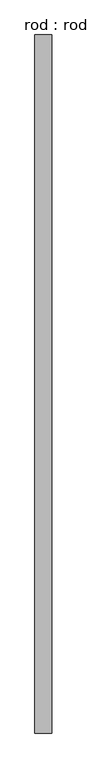
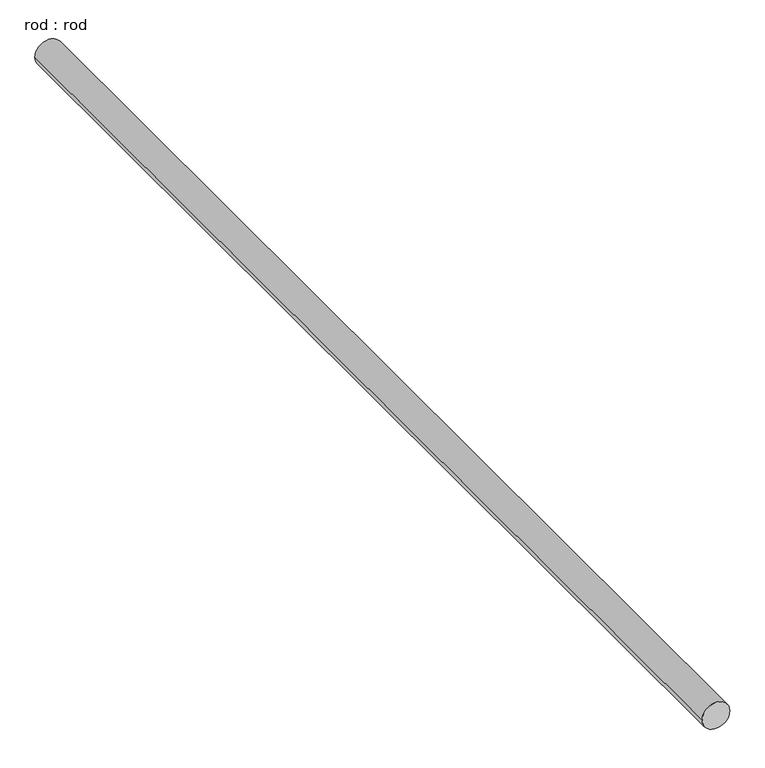
"""IFC4 building model written with IfcOpenShell, lengths in millimetres: proxy geometry, rod : rod."""

from ifc_helpers import new_model, si_unit, point, frame, frame_2d, origin, place, context, project, spatial, circle_curve, trimmed, segment, composite_curve, outline, extrude, source, transform, mapped, element, save


def rod_rod_f9913f1a(model_context):
    return source(origin(), model_context, "Body", "SweptSolid", [
        extrude(outline(composite_curve([segment(trimmed(circle_curve(frame_2d((0.0108462, 0.0)), 200.0), [point((0.0108462, 200.0))], [point((0.0108462, -200.0))], False, "CARTESIAN"), True, "CONTINUOUS"), segment(trimmed(circle_curve(frame_2d((0.0108462, 0.0)), 200.0), [point((0.0108462, -200.0))], [point((0.0108462, 200.0))], False, "CARTESIAN"), True, "CONTINUOUS")], self_intersect=False)), frame((0.0, -4271.0806992, 0.0), z_axis=(0.0, 1.0, 0.0), x_axis=(0.0, 0.0, 1.0)), (0.0, 0.0, 1.0), 16727.6186291),
    ])


if __name__ == "__main__":
    model = new_model("IFC4")
    model_context = context("Model", 3, world=origin())
    ifc_project = project(units=[si_unit("LENGTHUNIT", "METRE", prefix="MILLI")], contexts=[model_context])
    site = spatial("IfcSite", under=ifc_project)
    building = spatial("IfcBuilding", under=site)
    placement = place(None, origin())
    rod_rod_shape = rod_rod_f9913f1a(model_context)
    element("IfcBuildingElementProxy", 1, Name="rod : rod", ObjectType="rod : rod", at=placement, inside=building, context=model_context, shape_type="MappedRepresentation", body=[
        mapped(rod_rod_shape, transform((0.0, 0.0, 0.0), x_axis=(1.0, 0.0, 0.0), y_axis=(0.0, 1.0, 0.0), z_axis=(0.0, 0.0, 1.0))),
    ])
    save(model, "model.ifc")

# Revit data of these elements
# Type "rod : rod"
#   Default Elevation = 0
